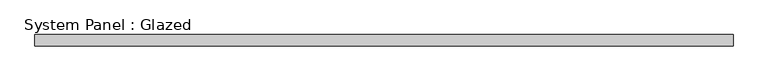
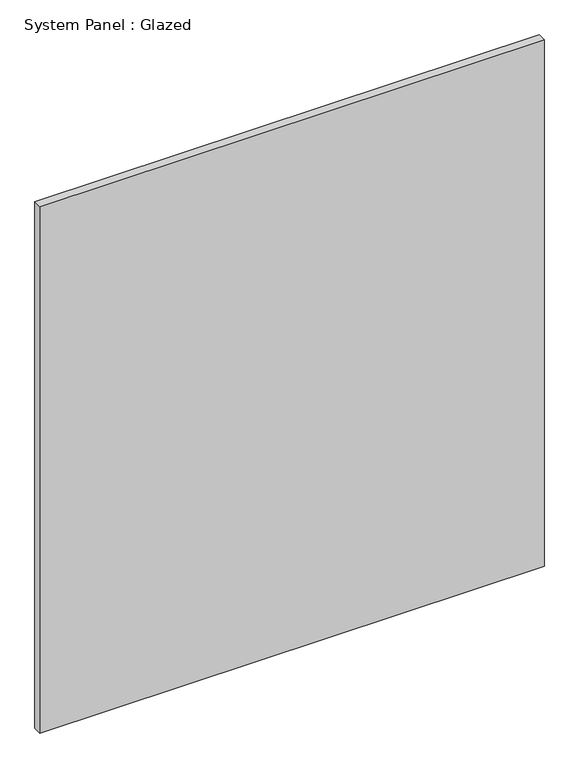
"""IFC4 building model written with IfcOpenShell, lengths in millimetres: plate geometry, System Panel : Glazed."""

from ifc_helpers import new_model, si_unit, origin, origin_with_axes, place, context, project, spatial, polyline, outline, extrude, source, transform, mapped, element, save


def system_panel_glazed_3ad970c3(model_context):
    return source(origin(), model_context, "Body", "SweptSolid", [
        extrude(outline(polyline([(770.0465291, 24.5), (-770.0465291, 24.5), (-770.0465291, 49.5), (770.0465291, 49.5), (770.0465291, 24.5)])), origin_with_axes(), (0.0, 0.0, 1.0), 1699.4222628),
    ])


if __name__ == "__main__":
    model = new_model("IFC4")
    model_context = context("Model", 3, world=origin())
    ifc_project = project(units=[si_unit("LENGTHUNIT", "METRE", prefix="MILLI")], contexts=[model_context])
    site = spatial("IfcSite", under=ifc_project)
    building = spatial("IfcBuilding", under=site)
    placement = place(None, origin())
    system_panel_glazed_shape = system_panel_glazed_3ad970c3(model_context)
    element("IfcPlate", 1, ObjectType="System Panel : Glazed", at=placement, inside=building, context=model_context, shape_type="MappedRepresentation", body=[
        mapped(system_panel_glazed_shape, transform((0.0, 0.0, 0.0), x_axis=(1.0, 0.0, 0.0), y_axis=(0.0, 1.0, 0.0), z_axis=(0.0, 0.0, 1.0))),
    ])
    save(model, "model.ifc")

# Revit data of these elements
# Element 1 (IfcPlate, "System Panel : Glazed")
#   Materials on its faces: "Glass"
# Materials
#   "Glass": class "Glass", colour RGB 218 227 224, transparency 0.85, Description = "Soda Lime Glass", Cost = 0
